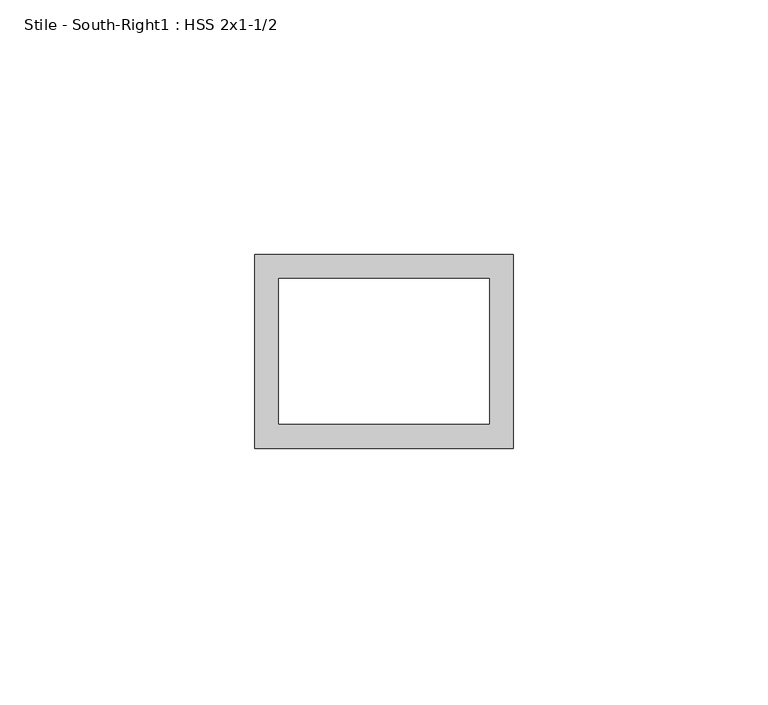
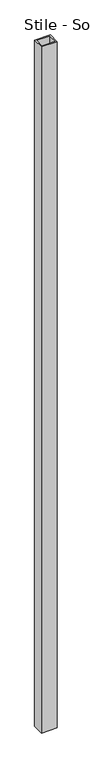
"""IFC4 building model written with IfcOpenShell, lengths in millimetres: proxy geometry, Stile - South-Right1 : HSS 2x1-1/2."""

import ifcopenshell
import ifcopenshell.guid

model = None  # the IFC model being written
_history = None  # IfcOwnerHistory: only IFC2X3 demands one
_inside = {}  # id of a spatial element -> (the spatial element, [elements in it])
_under = {}  # id of a project, library or spatial element -> (it, [spatial elements below it])
_declared = {}  # id of a project -> (the project, [libraries it declares])
_typed = {}  # id of a type object -> (the type object, [elements of that type])
_made_of = {}  # id of a material, layer set ... -> (it, [elements and type objects made of it])


def new_model(schema):
    """Start an empty IFC model of exactly this schema.

    Asked for "IFC4X3", IfcOpenShell would pick the latest addendum, in which some entities
    have other attributes; the version numbers below select the first issue.
    IFC2X3 requires an IfcOwnerHistory on every rooted entity: one is made here for all.
    """
    global model, _history
    if schema == "IFC4X3":
        model = ifcopenshell.file(schema_version=(4, 3, 0, 0))
    else:
        model = ifcopenshell.file(schema=schema)
    _inside.clear()
    _under.clear()
    _declared.clear()
    _typed.clear()
    _made_of.clear()
    _history = None
    if model.schema == "IFC2X3":
        org = make("IfcOrganization", Name="unknown")
        user = make(
            "IfcPersonAndOrganization",
            ThePerson=make("IfcPerson", FamilyName="unknown"),
            TheOrganization=org,
        )
        app = make(
            "IfcApplication",
            ApplicationDeveloper=org,
            Version="unknown",
            ApplicationFullName="unknown",
            ApplicationIdentifier="unknown",
        )
        _history = make(
            "IfcOwnerHistory",
            OwningUser=user,
            OwningApplication=app,
            ChangeAction="ADDED",
            CreationDate=0,
        )
    return model


def make(cls, **values):
    """One entity of the class cls with the attributes given. An attribute that is None is left unset."""
    return model.create_entity(
        cls, **{name: value for name, value in values.items() if value is not None}
    )


def rooted(cls, **values):
    """An entity with a GlobalId (a new one), such as an element, a storey or a relation."""
    return make(cls, GlobalId=ifcopenshell.guid.new(), OwnerHistory=_history, **values)


def si_unit(unit_type, name, prefix=None):
    """IfcSIUnit, for example si_unit("LENGTHUNIT", "METRE", prefix="MILLI")."""
    return make("IfcSIUnit", UnitType=unit_type, Prefix=prefix, Name=name)


def assignment(units):
    """IfcUnitAssignment: the units of a project."""
    return None if units is None else make("IfcUnitAssignment", Units=units)


def point(xyz):
    """IfcCartesianPoint."""
    return None if xyz is None else make("IfcCartesianPoint", Coordinates=xyz)


def direction(xyz):
    """IfcDirection."""
    return None if xyz is None else make("IfcDirection", DirectionRatios=xyz)


def frame(location, z_axis=None, x_axis=None):
    """IfcAxis2Placement3D, a coordinate frame: its origin and axes. An axis left out is left unset."""
    return make(
        "IfcAxis2Placement3D",
        Location=point(location),
        Axis=direction(z_axis),
        RefDirection=direction(x_axis),
    )


def origin():
    """The frame at (0, 0, 0) with its axes left unset."""
    return frame((0.0, 0.0, 0.0))


def place(relative_to, where):
    """IfcLocalPlacement: puts the frame where relative to a parent placement (None: the world)."""
    return make(
        "IfcLocalPlacement", PlacementRelTo=relative_to, RelativePlacement=where
    )


def context(
    kind, dimensions, precision=None, world=None, true_north=None, identifier=None
):
    """IfcGeometricRepresentationContext, for example the 3D "Model" context."""
    return make(
        "IfcGeometricRepresentationContext",
        ContextIdentifier=identifier,
        ContextType=kind,
        CoordinateSpaceDimension=dimensions,
        Precision=precision,
        WorldCoordinateSystem=world,
        TrueNorth=true_north,
    )


def project(units=None, contexts=None):
    """IfcProject with its units and contexts."""
    return rooted(
        "IfcProject",
        Name="project",
        RepresentationContexts=contexts,
        UnitsInContext=assignment(units),
    )


def spatial(cls, under=None, at=None, **own):
    """A site, building, storey or space (cls), placed at a placement, below another one or the project."""
    s = rooted(cls, ObjectPlacement=at, **own)
    if under is not None:
        _under.setdefault(under.id(), (under, []))[1].append(s)
    return s


def polyline(points):
    """IfcPolyline through the points."""
    return make("IfcPolyline", Points=[point(p) for p in points])


def outline(outer, holes=None, kind="AREA"):
    """IfcArbitraryClosedProfileDef: a profile drawn as a closed curve; with holes, ...WithVoids."""
    if holes is None:
        return make("IfcArbitraryClosedProfileDef", ProfileType=kind, OuterCurve=outer)
    return make(
        "IfcArbitraryProfileDefWithVoids",
        ProfileType=kind,
        OuterCurve=outer,
        InnerCurves=holes,
    )


def extrude(swept, where, along, depth):
    """IfcExtrudedAreaSolid: the profile swept, set in the frame where, extruded along a direction by depth."""
    return make(
        "IfcExtrudedAreaSolid",
        SweptArea=swept,
        Position=where,
        ExtrudedDirection=direction(along),
        Depth=depth,
    )


def shape(context_of_items, identifier, shape_type, items):
    """IfcShapeRepresentation: the items that make up one representation, for example the "Body"."""
    return make(
        "IfcShapeRepresentation",
        ContextOfItems=context_of_items,
        RepresentationIdentifier=identifier,
        RepresentationType=shape_type,
        Items=items,
    )


def source(mapping_origin, context_of_items, identifier, shape_type, items):
    """IfcRepresentationMap: a shape defined once, which mapped items show again and again."""
    return make(
        "IfcRepresentationMap",
        MappingOrigin=mapping_origin,
        MappedRepresentation=shape(context_of_items, identifier, shape_type, items),
    )


def transform(
    local_origin,
    x_axis=None,
    y_axis=None,
    z_axis=None,
    scale=None,
    scale2=None,
    scale3=None,
    uniform=True,
):
    """IfcCartesianTransformationOperator3D, or its non-uniform kind. x_axis, y_axis, z_axis: its Axis1, 2, 3."""
    if uniform:
        return make(
            "IfcCartesianTransformationOperator3D",
            Axis1=direction(x_axis),
            Axis2=direction(y_axis),
            LocalOrigin=point(local_origin),
            Scale=scale,
            Axis3=direction(z_axis),
        )
    return make(
        "IfcCartesianTransformationOperator3DnonUniform",
        Axis1=direction(x_axis),
        Axis2=direction(y_axis),
        LocalOrigin=point(local_origin),
        Scale=scale,
        Axis3=direction(z_axis),
        Scale2=scale2,
        Scale3=scale3,
    )


def mapped(mapping_source, mapping_target):
    """IfcMappedItem: shows the shape of a source again, moved by a transform."""
    return make(
        "IfcMappedItem", MappingSource=mapping_source, MappingTarget=mapping_target
    )


def made_of(thing, what):
    """Note that an element or type object is made of a material, layer set ...; save() writes the relation."""
    if what is not None:
        _made_of.setdefault(what.id(), (what, []))[1].append(thing)
    return thing


def element(
    cls,
    number,
    at=None,
    inside=None,
    cuts=None,
    type_object=None,
    material=None,
    context=None,
    identifier="Body",
    shape_type=None,
    held_by="IfcProductDefinitionShape",
    body=None,
    shapes=None,
    **own,
):
    """One element of the class cls, such as IfcWall. Its Tag is "e" and its number.

    at: its placement. inside: the storey or other place that contains it. cuts: it is an
    opening in that element (IfcRelVoidsElement). A single representation is given by context,
    identifier, shape_type and body (its items); several are given by shapes. held_by: the class
    of the entity that holds the representations. save() writes the other relations.
    """
    e = rooted(cls, Tag="e%d" % number, ObjectPlacement=at, **own)
    if body is not None:
        shapes = [shape(context, identifier, shape_type, body)]
    if shapes is not None:
        e.Representation = make(held_by, Representations=shapes)
    if inside is not None:
        _inside.setdefault(inside.id(), (inside, []))[1].append(e)
    if cuts is not None:
        rooted(
            "IfcRelVoidsElement", RelatingBuildingElement=cuts, RelatedOpeningElement=e
        )
    if type_object is not None:
        _typed.setdefault(type_object.id(), (type_object, []))[1].append(e)
    return made_of(e, material)


def aggregate(whole, parts):
    """IfcRelAggregates: a whole, such as a stair, and the parts it consists of."""
    return rooted("IfcRelAggregates", RelatingObject=whole, RelatedObjects=parts)


def save(model, path):
    """Write the relations noted so far, then the file.

    IfcRelAggregates (storeys below a building ...), IfcRelContainedInSpatialStructure (elements
    in a storey), IfcRelDefinesByType, IfcRelAssociatesMaterial and IfcRelDeclares: one each for
    every whole, place, type object, material and project.
    """
    for whole, parts in _under.values():
        aggregate(whole, parts)
    for where, things in _inside.values():
        rooted(
            "IfcRelContainedInSpatialStructure",
            RelatedElements=things,
            RelatingStructure=where,
        )
    for kind, things in _typed.values():
        rooted("IfcRelDefinesByType", RelatedObjects=things, RelatingType=kind)
    for what, things in _made_of.values():
        rooted("IfcRelAssociatesMaterial", RelatedObjects=things, RelatingMaterial=what)
    for by, libraries in _declared.values():
        rooted("IfcRelDeclares", RelatingContext=by, RelatedDefinitions=libraries)
    model.write(path)


def stile_south_right1_hss_2x1_1_2_42ef625e(model_context):
    return source(origin(), model_context, "Body", "SweptSolid", [
        extrude(outline(polyline([(587365.8934739, -536263.6038841), (587416.6934739, -536263.6038841), (587416.6934739, -536301.7038841), (587365.8934739, -536301.7038841), (587365.8934739, -536263.6038841)]), holes=[polyline([(587370.6559739, -536268.3663841), (587370.6559739, -536296.9413841), (587411.9309739, -536296.9413841), (587411.9309739, -536268.3663841), (587370.6559739, -536268.3663841)])]), frame((0.0, 0.0, 50.8), z_axis=(0.0, 0.0, 1.0), x_axis=(1.0, 0.0, 0.0)), (0.0, 0.0, 1.0), 2349.5),
    ])


if __name__ == "__main__":
    model = new_model("IFC4")
    model_context = context("Model", 3, world=origin())
    ifc_project = project(units=[si_unit("LENGTHUNIT", "METRE", prefix="MILLI")], contexts=[model_context])
    site = spatial("IfcSite", under=ifc_project)
    building = spatial("IfcBuilding", under=site)
    placement = place(None, origin())
    stile_south_right1_hss_2x1_1_2_shape = stile_south_right1_hss_2x1_1_2_42ef625e(model_context)
    element("IfcBuildingElementProxy", 1, Name="Stile - South-Right1 : HSS 2x1-1/2", ObjectType="Stile - South-Right1 : HSS 2x1-1/2", at=placement, inside=building, context=model_context, shape_type="MappedRepresentation", body=[
        mapped(stile_south_right1_hss_2x1_1_2_shape, transform((0.0, 0.0, 0.0), x_axis=(1.0, 0.0, 0.0), y_axis=(0.0, 1.0, 0.0), z_axis=(0.0, 0.0, 1.0))),
    ])
    save(model, "model.ifc")

# Revit data of these elements
# Element 1 (IfcBuildingElementProxy, "Stile - South-Right1 : HSS 2x1-1/2")
#   Materials on its faces: "1-1/2\"X2\" GALV. STL HSS TUBING"
# Materials
#   "1-1/2\"X2\" GALV. STL HSS TUBING": class "Generic", colour RGB 211 211 207, transparency 0, Cost = 0
